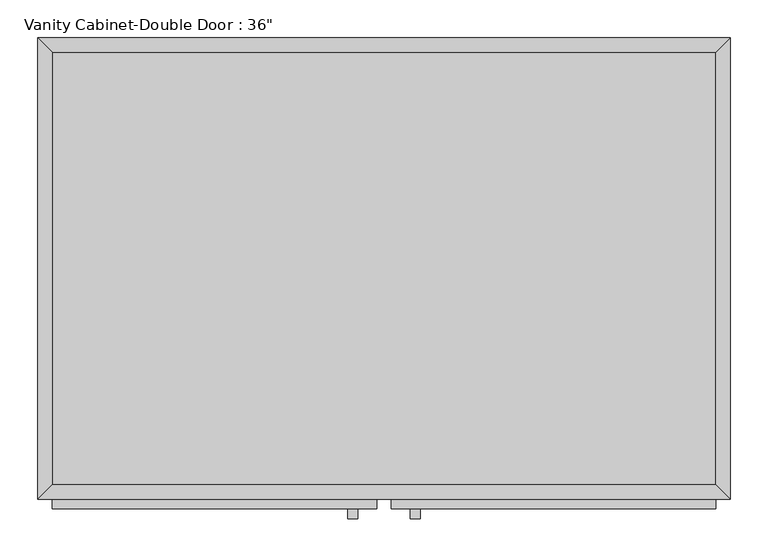
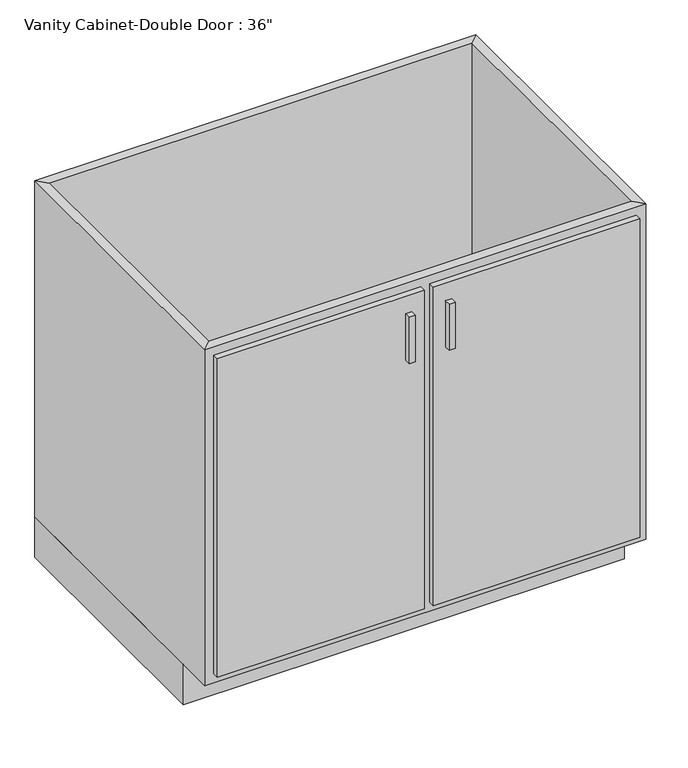
"""IFC4 building model written with IfcOpenShell, lengths in millimetres: furniture geometry."""

from ifc_helpers import new_model, si_unit, frame, origin, origin_with_axes, place, context, project, spatial, polyline, outline, extrude, faceted_brep, source, transform, mapped, element, save


def furniture_828f600b(model_context):
    return source(origin(), model_context, "Body", "SolidModel", [
        extrude(outline(polyline([(-16.1872951, -635.0), (-28.8872951, -635.0), (-28.8872951, -622.3), (-16.1872951, -622.3), (-16.1872951, -635.0)])), frame((0.0, 0.0, 666.75), z_axis=(0.0, 0.0, 1.0), x_axis=(1.0, 0.0, 0.0)), (0.0, 0.0, 1.0), 101.6),
        extrude(outline(polyline([(66.3627049, -635.0), (53.6627049, -635.0), (53.6627049, -622.3), (66.3627049, -622.3), (66.3627049, -635.0)])), frame((0.0, 0.0, 666.75), z_axis=(0.0, 0.0, 1.0), x_axis=(1.0, 0.0, 0.0)), (0.0, 0.0, 1.0), 101.6),
        extrude(outline(polyline([(9.2127049, -622.3), (-419.4122951, -622.3), (-419.4122951, -609.6), (9.2127049, -609.6), (9.2127049, -622.3)])), frame((0.0, 0.0, 107.95), z_axis=(0.0, 0.0, 1.0), x_axis=(1.0, 0.0, 0.0)), (0.0, 0.0, 1.0), 698.5),
        extrude(outline(polyline([(456.8877049, -622.3), (28.2627049, -622.3), (28.2627049, -609.6), (456.8877049, -609.6), (456.8877049, -622.3)])), frame((0.0, 0.0, 107.95), z_axis=(0.0, 0.0, 1.0), x_axis=(1.0, 0.0, 0.0)), (0.0, 0.0, 1.0), 698.5),
        extrude(outline(polyline([(456.8877049, -19.05), (456.8877049, -590.55), (-419.4122951, -590.55), (-419.4122951, -19.05), (456.8877049, -19.05)])), frame((0.0, 0.0, 88.9), z_axis=(0.0, 0.0, 1.0), x_axis=(1.0, 0.0, 0.0)), (0.0, 0.0, 1.0), 19.05),
        faceted_brep([(456.8877049, -590.55, 825.5), (456.8877049, -590.55, 88.9), (-419.4122951, -590.55, 88.9), (-419.4122951, -590.55, 825.5), (475.9377049, -609.6, 825.5), (-438.4622951, -609.6, 825.5), (475.9377049, -609.6, 88.9), (-438.4622951, -609.6, 88.9), (-419.4122951, -19.05, 88.9), (-419.4122951, -19.05, 825.5), (-438.4622951, 0.0, 825.5), (-438.4622951, 0.0, 88.9), (456.8877049, -19.05, 88.9), (456.8877049, -19.05, 825.5), (475.9377049, 0.0, 825.5), (475.9377049, 0.0, 88.9)], [[[0, 1, 2, 3]], [[4, 0, 3, 5]], [[6, 4, 5, 7]], [[1, 6, 7, 2]], [[3, 2, 8, 9]], [[5, 3, 9, 10]], [[7, 5, 10, 11]], [[2, 7, 11, 8]], [[9, 8, 12, 13]], [[10, 9, 13, 14]], [[11, 10, 14, 15]], [[8, 11, 15, 12]], [[13, 12, 1, 0]], [[14, 13, 0, 4]], [[15, 14, 4, 6]], [[12, 15, 6, 1]]]),
        extrude(outline(polyline([(475.9377049, 0.0), (475.9377049, -533.4), (-438.4622951, -533.4), (-438.4622951, 0.0), (475.9377049, 0.0)])), origin_with_axes(), (0.0, 0.0, 1.0), 88.9),
    ])


if __name__ == "__main__":
    model = new_model("IFC4")
    model_context = context("Model", 3, world=origin())
    ifc_project = project(units=[si_unit("LENGTHUNIT", "METRE", prefix="MILLI")], contexts=[model_context])
    site = spatial("IfcSite", under=ifc_project)
    building = spatial("IfcBuilding", under=site)
    placement = place(None, origin())
    furniture_shape = furniture_828f600b(model_context)
    element("IfcFurniture", 1, ObjectType="Vanity Cabinet-Double Door : 36\"", at=placement, inside=building, context=model_context, shape_type="MappedRepresentation", body=[
        mapped(furniture_shape, transform((0.0, 0.0, 0.0), x_axis=(1.0, 0.0, 0.0), y_axis=(0.0, 1.0, 0.0), z_axis=(0.0, 0.0, 1.0))),
    ])
    save(model, "model.ifc")

# Revit data of these elements
# Type "Vanity Cabinet-Double Door : 36\""
#   Finish = "Cabinetry"
#   Finish = "Cabinetry"
#   Assembly Code = "C1030410"
#   Depth = 2' - 0"
#   Height = 2' - 8 1/2"
#   Toe Depth = 0' - 3"
#   Toe Height = 0' - 3 1/2"
#   Width = 3' - 0"
#   Cabinet Material = none
#   Door/Drawer Material = none
#   Handle Material = none
# Element 1 (IfcFurniture, "Vanity Cabinet-Double Door : 36\"")
#   Materials on its faces: "CASEWORK"
# Materials
#   "CASEWORK": class "Generic", colour RGB 181 181 181, transparency 0, Cost = 0
